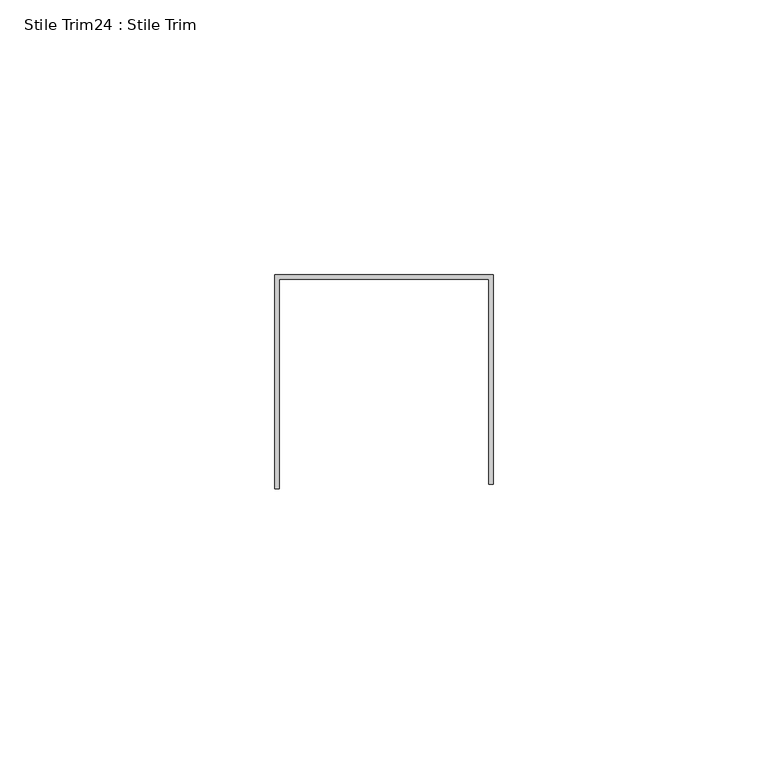
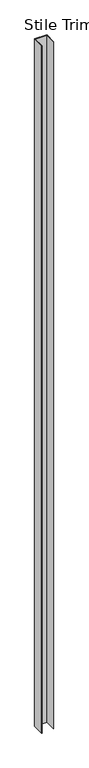
"""IFC4 building model written with IfcOpenShell, lengths in millimetres: proxy geometry, Stile Trim24 : Stile Trim."""

from ifc_helpers import new_model, si_unit, frame, origin, place, context, project, spatial, polyline, outline, extrude, source, transform, mapped, element, save


def stile_trim24_stile_trim_ecce4863(model_context):
    return source(origin(), model_context, "Body", "SweptSolid", [
        extrude(outline(polyline([(587327.0060739, -534108.5789841), (587366.6808739, -534108.5789841), (587366.6808739, -534146.6789841), (587365.8934739, -534146.6789841), (587365.8934739, -534109.3663841), (587327.7934739, -534109.3663841), (587327.7934739, -534147.4663841), (587327.0060739, -534147.4663841), (587327.0060739, -534108.5789841)])), frame((0.0, 0.0, 50.8), z_axis=(0.0, 0.0, 1.0), x_axis=(1.0, 0.0, 0.0)), (0.0, 0.0, 1.0), 2350.3929688),
    ])


if __name__ == "__main__":
    model = new_model("IFC4")
    model_context = context("Model", 3, world=origin())
    ifc_project = project(units=[si_unit("LENGTHUNIT", "METRE", prefix="MILLI")], contexts=[model_context])
    site = spatial("IfcSite", under=ifc_project)
    building = spatial("IfcBuilding", under=site)
    placement = place(None, origin())
    stile_trim24_stile_trim_shape = stile_trim24_stile_trim_ecce4863(model_context)
    element("IfcBuildingElementProxy", 1, Name="Stile Trim24 : Stile Trim", ObjectType="Stile Trim24 : Stile Trim", at=placement, inside=building, context=model_context, shape_type="MappedRepresentation", body=[
        mapped(stile_trim24_stile_trim_shape, transform((0.0, 0.0, 0.0), x_axis=(1.0, 0.0, 0.0), y_axis=(0.0, 1.0, 0.0), z_axis=(0.0, 0.0, 1.0))),
    ])
    save(model, "model.ifc")

# Revit data of these elements
# Element 1 (IfcBuildingElementProxy, "Stile Trim24 : Stile Trim")
#   Materials on its faces: "EDGE TRIM BY MTL PANEL MFR."
# Materials
#   "EDGE TRIM BY MTL PANEL MFR.": class "Generic", colour RGB 239 242 240, transparency 0, Cost = 0
